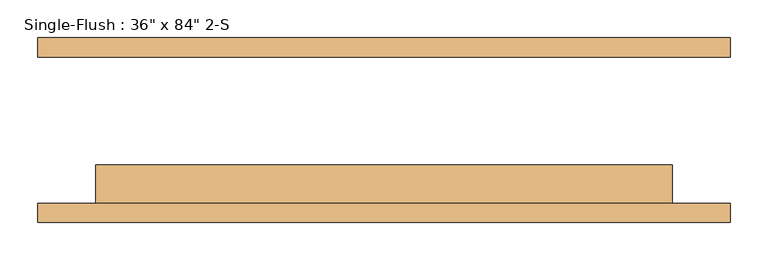
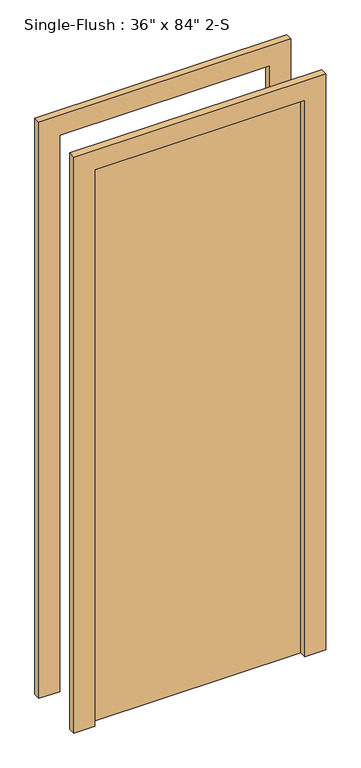
"""IFC4 building model written with IfcOpenShell, lengths in millimetres: door geometry."""

import ifcopenshell
import ifcopenshell.guid

model = None  # the IFC model being written
_history = None  # IfcOwnerHistory: only IFC2X3 demands one
_inside = {}  # id of a spatial element -> (the spatial element, [elements in it])
_under = {}  # id of a project, library or spatial element -> (it, [spatial elements below it])
_declared = {}  # id of a project -> (the project, [libraries it declares])
_typed = {}  # id of a type object -> (the type object, [elements of that type])
_made_of = {}  # id of a material, layer set ... -> (it, [elements and type objects made of it])


def new_model(schema):
    """Start an empty IFC model of exactly this schema.

    Asked for "IFC4X3", IfcOpenShell would pick the latest addendum, in which some entities
    have other attributes; the version numbers below select the first issue.
    IFC2X3 requires an IfcOwnerHistory on every rooted entity: one is made here for all.
    """
    global model, _history
    if schema == "IFC4X3":
        model = ifcopenshell.file(schema_version=(4, 3, 0, 0))
    else:
        model = ifcopenshell.file(schema=schema)
    _inside.clear()
    _under.clear()
    _declared.clear()
    _typed.clear()
    _made_of.clear()
    _history = None
    if model.schema == "IFC2X3":
        org = make("IfcOrganization", Name="unknown")
        user = make(
            "IfcPersonAndOrganization",
            ThePerson=make("IfcPerson", FamilyName="unknown"),
            TheOrganization=org,
        )
        app = make(
            "IfcApplication",
            ApplicationDeveloper=org,
            Version="unknown",
            ApplicationFullName="unknown",
            ApplicationIdentifier="unknown",
        )
        _history = make(
            "IfcOwnerHistory",
            OwningUser=user,
            OwningApplication=app,
            ChangeAction="ADDED",
            CreationDate=0,
        )
    return model


def make(cls, **values):
    """One entity of the class cls with the attributes given. An attribute that is None is left unset."""
    return model.create_entity(
        cls, **{name: value for name, value in values.items() if value is not None}
    )


def rooted(cls, **values):
    """An entity with a GlobalId (a new one), such as an element, a storey or a relation."""
    return make(cls, GlobalId=ifcopenshell.guid.new(), OwnerHistory=_history, **values)


def si_unit(unit_type, name, prefix=None):
    """IfcSIUnit, for example si_unit("LENGTHUNIT", "METRE", prefix="MILLI")."""
    return make("IfcSIUnit", UnitType=unit_type, Prefix=prefix, Name=name)


def assignment(units):
    """IfcUnitAssignment: the units of a project."""
    return None if units is None else make("IfcUnitAssignment", Units=units)


def point(xyz):
    """IfcCartesianPoint."""
    return None if xyz is None else make("IfcCartesianPoint", Coordinates=xyz)


def direction(xyz):
    """IfcDirection."""
    return None if xyz is None else make("IfcDirection", DirectionRatios=xyz)


def frame(location, z_axis=None, x_axis=None):
    """IfcAxis2Placement3D, a coordinate frame: its origin and axes. An axis left out is left unset."""
    return make(
        "IfcAxis2Placement3D",
        Location=point(location),
        Axis=direction(z_axis),
        RefDirection=direction(x_axis),
    )


def origin():
    """The frame at (0, 0, 0) with its axes left unset."""
    return frame((0.0, 0.0, 0.0))


def origin_with_axes():
    """The frame at (0, 0, 0) with the z axis (0, 0, 1) and the x axis (1, 0, 0) written out."""
    return frame((0.0, 0.0, 0.0), z_axis=(0.0, 0.0, 1.0), x_axis=(1.0, 0.0, 0.0))


def place(relative_to, where):
    """IfcLocalPlacement: puts the frame where relative to a parent placement (None: the world)."""
    return make(
        "IfcLocalPlacement", PlacementRelTo=relative_to, RelativePlacement=where
    )


def context(
    kind, dimensions, precision=None, world=None, true_north=None, identifier=None
):
    """IfcGeometricRepresentationContext, for example the 3D "Model" context."""
    return make(
        "IfcGeometricRepresentationContext",
        ContextIdentifier=identifier,
        ContextType=kind,
        CoordinateSpaceDimension=dimensions,
        Precision=precision,
        WorldCoordinateSystem=world,
        TrueNorth=true_north,
    )


def project(units=None, contexts=None):
    """IfcProject with its units and contexts."""
    return rooted(
        "IfcProject",
        Name="project",
        RepresentationContexts=contexts,
        UnitsInContext=assignment(units),
    )


def spatial(cls, under=None, at=None, **own):
    """A site, building, storey or space (cls), placed at a placement, below another one or the project."""
    s = rooted(cls, ObjectPlacement=at, **own)
    if under is not None:
        _under.setdefault(under.id(), (under, []))[1].append(s)
    return s


def polyline(points):
    """IfcPolyline through the points."""
    return make("IfcPolyline", Points=[point(p) for p in points])


def outline(outer, holes=None, kind="AREA"):
    """IfcArbitraryClosedProfileDef: a profile drawn as a closed curve; with holes, ...WithVoids."""
    if holes is None:
        return make("IfcArbitraryClosedProfileDef", ProfileType=kind, OuterCurve=outer)
    return make(
        "IfcArbitraryProfileDefWithVoids",
        ProfileType=kind,
        OuterCurve=outer,
        InnerCurves=holes,
    )


def extrude(swept, where, along, depth):
    """IfcExtrudedAreaSolid: the profile swept, set in the frame where, extruded along a direction by depth."""
    return make(
        "IfcExtrudedAreaSolid",
        SweptArea=swept,
        Position=where,
        ExtrudedDirection=direction(along),
        Depth=depth,
    )


def shape(context_of_items, identifier, shape_type, items):
    """IfcShapeRepresentation: the items that make up one representation, for example the "Body"."""
    return make(
        "IfcShapeRepresentation",
        ContextOfItems=context_of_items,
        RepresentationIdentifier=identifier,
        RepresentationType=shape_type,
        Items=items,
    )


def source(mapping_origin, context_of_items, identifier, shape_type, items):
    """IfcRepresentationMap: a shape defined once, which mapped items show again and again."""
    return make(
        "IfcRepresentationMap",
        MappingOrigin=mapping_origin,
        MappedRepresentation=shape(context_of_items, identifier, shape_type, items),
    )


def transform(
    local_origin,
    x_axis=None,
    y_axis=None,
    z_axis=None,
    scale=None,
    scale2=None,
    scale3=None,
    uniform=True,
):
    """IfcCartesianTransformationOperator3D, or its non-uniform kind. x_axis, y_axis, z_axis: its Axis1, 2, 3."""
    if uniform:
        return make(
            "IfcCartesianTransformationOperator3D",
            Axis1=direction(x_axis),
            Axis2=direction(y_axis),
            LocalOrigin=point(local_origin),
            Scale=scale,
            Axis3=direction(z_axis),
        )
    return make(
        "IfcCartesianTransformationOperator3DnonUniform",
        Axis1=direction(x_axis),
        Axis2=direction(y_axis),
        LocalOrigin=point(local_origin),
        Scale=scale,
        Axis3=direction(z_axis),
        Scale2=scale2,
        Scale3=scale3,
    )


def mapped(mapping_source, mapping_target):
    """IfcMappedItem: shows the shape of a source again, moved by a transform."""
    return make(
        "IfcMappedItem", MappingSource=mapping_source, MappingTarget=mapping_target
    )


def made_of(thing, what):
    """Note that an element or type object is made of a material, layer set ...; save() writes the relation."""
    if what is not None:
        _made_of.setdefault(what.id(), (what, []))[1].append(thing)
    return thing


def element(
    cls,
    number,
    at=None,
    inside=None,
    cuts=None,
    type_object=None,
    material=None,
    context=None,
    identifier="Body",
    shape_type=None,
    held_by="IfcProductDefinitionShape",
    body=None,
    shapes=None,
    **own,
):
    """One element of the class cls, such as IfcWall. Its Tag is "e" and its number.

    at: its placement. inside: the storey or other place that contains it. cuts: it is an
    opening in that element (IfcRelVoidsElement). A single representation is given by context,
    identifier, shape_type and body (its items); several are given by shapes. held_by: the class
    of the entity that holds the representations. save() writes the other relations.
    """
    e = rooted(cls, Tag="e%d" % number, ObjectPlacement=at, **own)
    if body is not None:
        shapes = [shape(context, identifier, shape_type, body)]
    if shapes is not None:
        e.Representation = make(held_by, Representations=shapes)
    if inside is not None:
        _inside.setdefault(inside.id(), (inside, []))[1].append(e)
    if cuts is not None:
        rooted(
            "IfcRelVoidsElement", RelatingBuildingElement=cuts, RelatedOpeningElement=e
        )
    if type_object is not None:
        _typed.setdefault(type_object.id(), (type_object, []))[1].append(e)
    return made_of(e, material)


def aggregate(whole, parts):
    """IfcRelAggregates: a whole, such as a stair, and the parts it consists of."""
    return rooted("IfcRelAggregates", RelatingObject=whole, RelatedObjects=parts)


def save(model, path):
    """Write the relations noted so far, then the file.

    IfcRelAggregates (storeys below a building ...), IfcRelContainedInSpatialStructure (elements
    in a storey), IfcRelDefinesByType, IfcRelAssociatesMaterial and IfcRelDeclares: one each for
    every whole, place, type object, material and project.
    """
    for whole, parts in _under.values():
        aggregate(whole, parts)
    for where, things in _inside.values():
        rooted(
            "IfcRelContainedInSpatialStructure",
            RelatedElements=things,
            RelatingStructure=where,
        )
    for kind, things in _typed.values():
        rooted("IfcRelDefinesByType", RelatedObjects=things, RelatingType=kind)
    for what, things in _made_of.values():
        rooted("IfcRelAssociatesMaterial", RelatedObjects=things, RelatingMaterial=what)
    for by, libraries in _declared.values():
        rooted("IfcRelDeclares", RelatingContext=by, RelatedDefinitions=libraries)
    model.write(path)


def door_e38c93b8(model_context):
    return source(origin(), model_context, "Body", "SweptSolid", [
        extrude(outline(polyline([(2209.8, -457.2), (0.0, -457.2), (0.0, -381.0), (2133.6, -381.0), (2133.6, 381.0), (0.0, 381.0), (0.0, 457.2), (2209.8, 457.2), (2209.8, -457.2)])), frame((0.0, -122.2375, 0.0), z_axis=(0.0, 1.0, 0.0), x_axis=(0.0, 0.0, 1.0)), (0.0, 0.0, 1.0), 25.4),
        extrude(outline(polyline([(2209.8, 457.2), (2209.8, -457.2), (0.0, -457.2), (0.0, -381.0), (2133.6, -381.0), (2133.6, 381.0), (0.0, 381.0), (0.0, 457.2), (2209.8, 457.2)])), frame((0.0, 96.8375, 0.0), z_axis=(0.0, 1.0, 0.0), x_axis=(0.0, 0.0, 1.0)), (0.0, 0.0, 1.0), 25.4),
        extrude(outline(polyline([(381.0, -46.0375), (381.0, -96.8375), (-381.0, -96.8375), (-381.0, -46.0375), (381.0, -46.0375)])), origin_with_axes(), (0.0, 0.0, 1.0), 2133.6),
    ])


if __name__ == "__main__":
    model = new_model("IFC4")
    model_context = context("Model", 3, world=origin())
    ifc_project = project(units=[si_unit("LENGTHUNIT", "METRE", prefix="MILLI")], contexts=[model_context])
    site = spatial("IfcSite", under=ifc_project)
    building = spatial("IfcBuilding", under=site)
    placement = place(None, origin())
    door_shape = door_e38c93b8(model_context)
    element("IfcDoor", 1, ObjectType="Single-Flush : 36\" x 84\" 2-S", at=placement, inside=building, context=model_context, shape_type="MappedRepresentation", body=[
        mapped(door_shape, transform((0.0, 0.0, 0.0), x_axis=(1.0, 0.0, 0.0), y_axis=(0.0, 1.0, 0.0), z_axis=(0.0, 0.0, 1.0))),
    ])
    save(model, "model.ifc")

# Revit data of these elements
# Type "Single-Flush : 36\" x 84\" 2-S"
#   Type Mark = "57"
#   Assembly Code = "C1020"
#   Thickness = 0' - 2"
#   Height = 7' - 0"
#   Trim Projection Ext = 0' - 1"
#   Trim Projection Int = 0' - 1"
#   Trim Width = 0' - 3"
#   Width = 2' - 6"
#   Door Material = Door - Panel
#   Frame Material = Door - Frame
#   Wall Closure = (empty or 0)
# Element 1 (IfcDoor, "Single-Flush : 36\" x 84\" 2-S")
#   Materials on its faces: "Door - Frame", "Door - Panel"
# Materials
#   "Door - Panel": class "Wood", colour RGB 227 170 128, transparency 0, Cost = 0
#   "Door - Frame": class "Miscellaneous", colour RGB 153 76 43, transparency 0, Cost = 0
